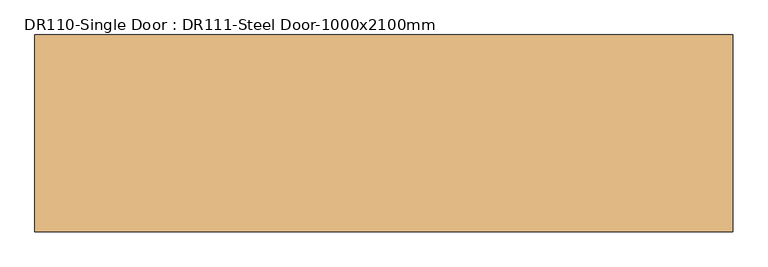
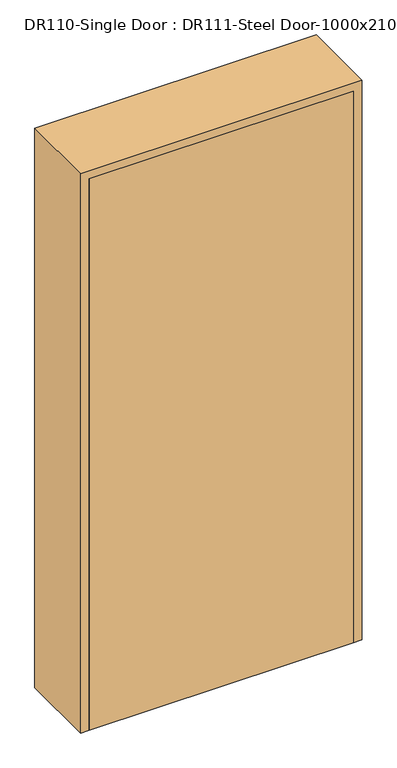
"""IFC4 building model written with IfcOpenShell, lengths in millimetres: door geometry, DR110-Single Door : DR111-Steel Door-1000x2100mm."""

from ifc_helpers import new_model, si_unit, origin, origin_with_axes, place, context, project, spatial, polyline, outline, extrude, faceted_brep, source, transform, mapped, element, save


def dr110_single_door_dr111_steel_door_1000x2100mm_481420e4(model_context):
    return source(origin(), model_context, "Body", "SolidModel", [
        extrude(outline(polyline([(470.0, -141.0), (-470.0, -141.0), (-470.0, -106.0), (470.0, -106.0), (470.0, -141.0)])), origin_with_axes(), (0.0, 0.0, 1.0), 2070.0),
        faceted_brep([(470.0, -141.0, 0.0), (470.0, -106.0, 0.0), (450.0, -106.0, 0.0), (450.0, 106.0, 0.0), (470.0, 106.0, 0.0), (470.0, 141.0, 0.0), (500.0, 141.0, 0.0), (500.0, -141.0, 0.0), (500.0, -141.0, 2100.0), (-500.0, -141.0, 2100.0), (-500.0, -141.0, 0.0), (-470.0, -141.0, 0.0), (-470.0, -141.0, 2070.0), (470.0, -141.0, 2070.0), (500.0, 141.0, 2100.0), (470.0, 141.0, 2070.0), (-470.0, 141.0, 2070.0), (-470.0, 141.0, 0.0), (-500.0, 141.0, 0.0), (-500.0, 141.0, 2100.0), (470.0, 106.0, 2070.0), (450.0, 106.0, 2050.0), (-450.0, 106.0, 2050.0), (-450.0, 106.0, 0.0), (-470.0, 106.0, 0.0), (-470.0, 106.0, 2070.0), (450.0, -106.0, 2050.0), (470.0, -106.0, 2070.0), (-470.0, -106.0, 2070.0), (-470.0, -106.0, 0.0), (-450.0, -106.0, 0.0), (-450.0, -106.0, 2050.0)], [[[0, 1, 2, 3, 4, 5, 6, 7]], [[7, 8, 9, 10, 11, 12, 13, 0]], [[6, 14, 8, 7]], [[5, 15, 16, 17, 18, 19, 14, 6]], [[4, 20, 15, 5]], [[3, 21, 22, 23, 24, 25, 20, 4]], [[2, 26, 21, 3]], [[1, 27, 28, 29, 30, 31, 26, 2]], [[0, 13, 27, 1]], [[12, 11, 29, 28]], [[11, 10, 18, 17, 24, 23, 30, 29]], [[19, 18, 10, 9]], [[25, 24, 17, 16]], [[31, 30, 23, 22]], [[14, 19, 9, 8]], [[20, 25, 16, 15]], [[26, 31, 22, 21]], [[13, 12, 28, 27]]]),
    ])


if __name__ == "__main__":
    model = new_model("IFC4")
    model_context = context("Model", 3, world=origin())
    ifc_project = project(units=[si_unit("LENGTHUNIT", "METRE", prefix="MILLI")], contexts=[model_context])
    site = spatial("IfcSite", under=ifc_project)
    building = spatial("IfcBuilding", under=site)
    placement = place(None, origin())
    dr110_single_door_dr111_steel_door_1000x2100mm_shape = dr110_single_door_dr111_steel_door_1000x2100mm_481420e4(model_context)
    element("IfcDoor", 1, ObjectType="DR110-Single Door : DR111-Steel Door-1000x2100mm", at=placement, inside=building, context=model_context, shape_type="MappedRepresentation", body=[
        mapped(dr110_single_door_dr111_steel_door_1000x2100mm_shape, transform((0.0, 0.0, 0.0), x_axis=(1.0, 0.0, 0.0), y_axis=(0.0, 1.0, 0.0), z_axis=(0.0, 0.0, 1.0))),
    ])
    save(model, "model.ifc")

# Revit data of these elements
# Type "DR110-Single Door : DR111-Steel Door-1000x2100mm"
#   Description = "DSDSSD"
#   Type Mark = "SD"
#   Analytic Construction = "<None>"
#   프레임 투영 외부. = 25 mm
#   프레임 투영 내부. = 25 mm
#   프레임 폭 = 75 mm
#   Height = 2100 mm
#   Width = 1000 mm
#   Define Thermal Properties by = 1
#   문 패널 = SD1 문 패널
#   문 프레임 = A04AQ098-00002_Steel Door_non FP_single
#   Function = (empty or 0)
#   Wall Closure = (empty or 0)
# Element 1 (IfcDoor, "DR110-Single Door : DR111-Steel Door-1000x2100mm")
#   Materials on its faces: "A04AQ098-00002_Steel Door_non FP_single", "SD1 문 패널"
# Materials
#   "SD1 문 패널": class "금속", colour RGB 247 247 247, transparency 0, Description = "STEEL DOOR (1000Wx2100H)"
#   "A04AQ098-00002_Steel Door_non FP_single": class "금속", colour RGB 247 247 247, transparency 0, Description = "Steel Door", W00) Work Master Code = "A04AQ098-00002", W01) Work Master_Lv1 = "Finishing Work", W02) Work Master_Lv2 = "Door & Window Work", W03) Work Master_Spec.1 = "Steel Door w/ Steel Frame", W04) Work Master_Spec.2 = "Fire Protective Rating: N/A, Single Door", W05) Work Master_Spec.3 = "w/ Hardware & Accessories", Cost = 0
